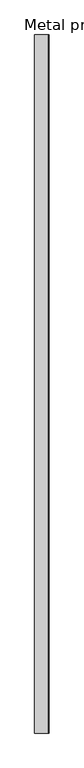
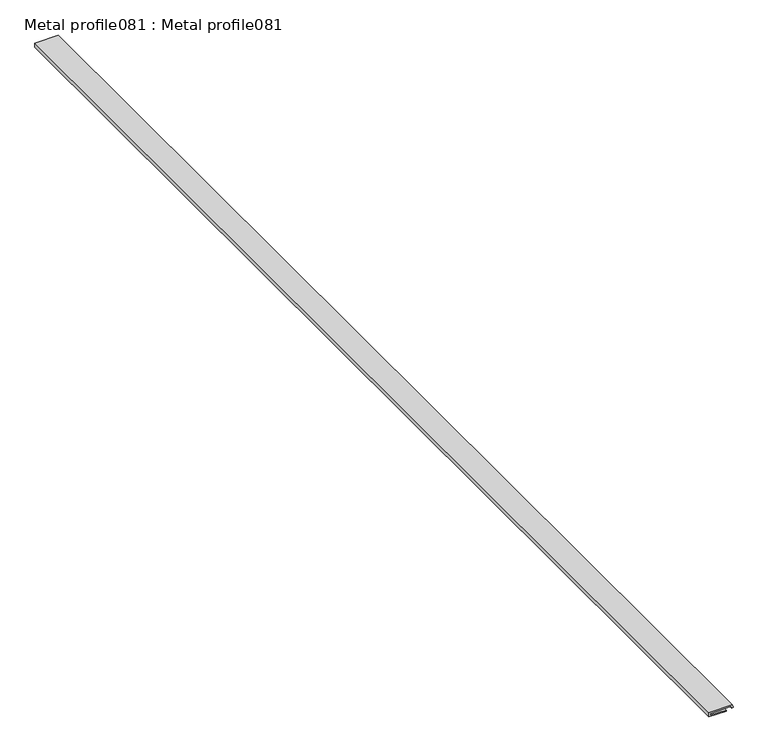
"""IFC4 building model written with IfcOpenShell, lengths in millimetres: proxy geometry, Metal profile081 : Metal profile081."""

from ifc_helpers import new_model, si_unit, frame, origin, place, context, project, spatial, polyline, outline, extrude, source, transform, mapped, element, save


def metal_profile081_metal_profile081_cc68793d(model_context):
    return source(origin(), model_context, "Body", "SweptSolid", [
        extrude(outline(polyline([(40172.6132812, -7123.5799076), (40172.6132812, -7150.8474857), (40175.9203326, -7150.8474857), (40176.4624429, -7114.624178), (40172.8172405, -7113.4516003), (40173.4296875, -7111.547681), (40178.484375, -7113.1736576), (40177.890625, -7152.8474857), (40170.6132812, -7152.8474857), (40170.6132812, -7123.5799076), (40172.6132812, -7123.5799076)])), frame((0.0, 7982.1531721, 0.0), z_axis=(0.0, 1.0, 0.0), x_axis=(0.0, 0.0, 1.0)), (0.0, 0.0, 1.0), 2000.0),
    ])


if __name__ == "__main__":
    model = new_model("IFC4")
    model_context = context("Model", 3, world=origin())
    ifc_project = project(units=[si_unit("LENGTHUNIT", "METRE", prefix="MILLI")], contexts=[model_context])
    site = spatial("IfcSite", under=ifc_project)
    building = spatial("IfcBuilding", under=site)
    placement = place(None, origin())
    metal_profile081_metal_profile081_shape = metal_profile081_metal_profile081_cc68793d(model_context)
    element("IfcBuildingElementProxy", 1, Name="Metal profile081 : Metal profile081", ObjectType="Metal profile081 : Metal profile081", at=placement, inside=building, context=model_context, shape_type="MappedRepresentation", body=[
        mapped(metal_profile081_metal_profile081_shape, transform((0.0, 0.0, 0.0), x_axis=(1.0, 0.0, 0.0), y_axis=(0.0, 1.0, 0.0), z_axis=(0.0, 0.0, 1.0))),
    ])
    save(model, "model.ifc")

# Revit data of these elements
# Type "Metal profile081 : Metal profile081"
#   NameOverride = "Metal profile081"
# Element 1 (IfcBuildingElementProxy, "Metal profile081 : Metal profile081")
#   Materials on its faces: "ANGLE TRIM"
# Materials
#   "ANGLE TRIM": class "Unassigned", colour RGB 250 255 0, transparency 0
